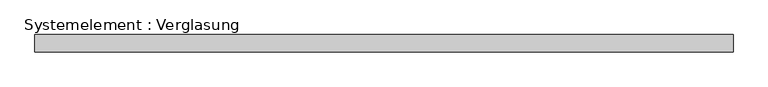
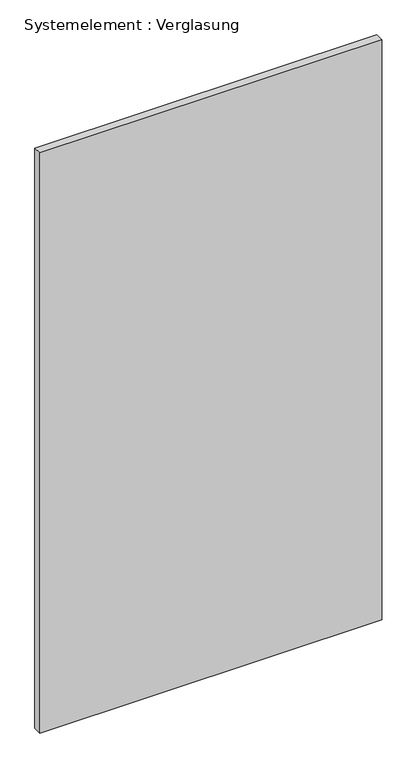
"""IFC4 building model written with IfcOpenShell, lengths in millimetres: plate geometry, Systemelement : Verglasung."""

from ifc_helpers import new_model, si_unit, origin, origin_with_axes, place, context, project, spatial, polyline, outline, extrude, source, transform, mapped, element, save


def systemelement_verglasung_f34c0457(model_context):
    return source(origin(), model_context, "Body", "SweptSolid", [
        extrude(outline(polyline([(605.0000002, -15.0), (-605.0000002, -15.0), (-605.0000002, 15.0), (605.0000002, 15.0), (605.0000002, -15.0)])), origin_with_axes(), (0.0, 0.0, 1.0), 2170.8558388),
    ])


if __name__ == "__main__":
    model = new_model("IFC4")
    model_context = context("Model", 3, world=origin())
    ifc_project = project(units=[si_unit("LENGTHUNIT", "METRE", prefix="MILLI")], contexts=[model_context])
    site = spatial("IfcSite", under=ifc_project)
    building = spatial("IfcBuilding", under=site)
    placement = place(None, origin())
    systemelement_verglasung_shape = systemelement_verglasung_f34c0457(model_context)
    element("IfcPlate", 1, ObjectType="Systemelement : Verglasung", at=placement, inside=building, context=model_context, shape_type="MappedRepresentation", body=[
        mapped(systemelement_verglasung_shape, transform((0.0, 0.0, 0.0), x_axis=(1.0, 0.0, 0.0), y_axis=(0.0, 1.0, 0.0), z_axis=(0.0, 0.0, 1.0))),
    ])
    save(model, "model.ifc")

# Revit data of these elements
# Type "Systemelement : Verglasung"
#   Construction Type Id = "GSP4R"
#   Analytic Construction = "1/8 Zoll Pilkington-Verglasung einfach"
#   Visual Light Transmittance = 0.9
#   Solar Heat Gain Coefficient = 0.86
#   Heat Transfer Coefficient (U) = 6.7069 W/(m²·K)
# Element 1 (IfcPlate, "Systemelement : Verglasung")
#   Materials on its faces: "Glas"
# Materials
#   "Glas": class "Glas", colour RGB 0 0 255, transparency 0.75, Comments = "Render-Darstellung nicht aktualisiert ", Cost = 0
